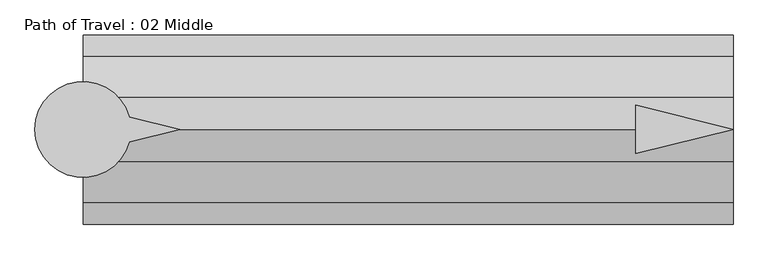
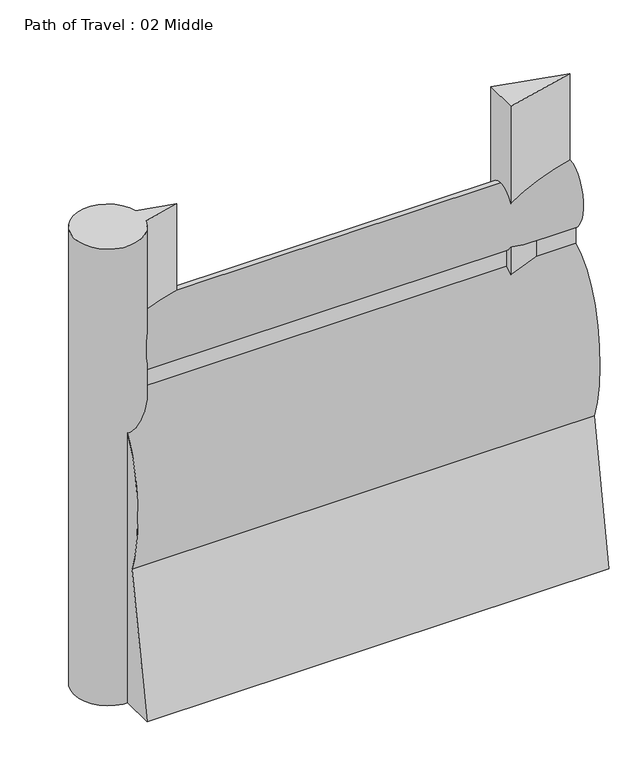
"""IFC4 building model written with IfcOpenShell, lengths in millimetres: proxy geometry, Path of Travel : 02 Middle."""

import ifcopenshell
import ifcopenshell.guid

model = None  # the IFC model being written
_history = None  # IfcOwnerHistory: only IFC2X3 demands one
_inside = {}  # id of a spatial element -> (the spatial element, [elements in it])
_under = {}  # id of a project, library or spatial element -> (it, [spatial elements below it])
_declared = {}  # id of a project -> (the project, [libraries it declares])
_typed = {}  # id of a type object -> (the type object, [elements of that type])
_made_of = {}  # id of a material, layer set ... -> (it, [elements and type objects made of it])


def new_model(schema):
    """Start an empty IFC model of exactly this schema.

    Asked for "IFC4X3", IfcOpenShell would pick the latest addendum, in which some entities
    have other attributes; the version numbers below select the first issue.
    IFC2X3 requires an IfcOwnerHistory on every rooted entity: one is made here for all.
    """
    global model, _history
    if schema == "IFC4X3":
        model = ifcopenshell.file(schema_version=(4, 3, 0, 0))
    else:
        model = ifcopenshell.file(schema=schema)
    _inside.clear()
    _under.clear()
    _declared.clear()
    _typed.clear()
    _made_of.clear()
    _history = None
    if model.schema == "IFC2X3":
        org = make("IfcOrganization", Name="unknown")
        user = make(
            "IfcPersonAndOrganization",
            ThePerson=make("IfcPerson", FamilyName="unknown"),
            TheOrganization=org,
        )
        app = make(
            "IfcApplication",
            ApplicationDeveloper=org,
            Version="unknown",
            ApplicationFullName="unknown",
            ApplicationIdentifier="unknown",
        )
        _history = make(
            "IfcOwnerHistory",
            OwningUser=user,
            OwningApplication=app,
            ChangeAction="ADDED",
            CreationDate=0,
        )
    return model


def make(cls, **values):
    """One entity of the class cls with the attributes given. An attribute that is None is left unset."""
    return model.create_entity(
        cls, **{name: value for name, value in values.items() if value is not None}
    )


def rooted(cls, **values):
    """An entity with a GlobalId (a new one), such as an element, a storey or a relation."""
    return make(cls, GlobalId=ifcopenshell.guid.new(), OwnerHistory=_history, **values)


def si_unit(unit_type, name, prefix=None):
    """IfcSIUnit, for example si_unit("LENGTHUNIT", "METRE", prefix="MILLI")."""
    return make("IfcSIUnit", UnitType=unit_type, Prefix=prefix, Name=name)


def assignment(units):
    """IfcUnitAssignment: the units of a project."""
    return None if units is None else make("IfcUnitAssignment", Units=units)


def point(xyz):
    """IfcCartesianPoint."""
    return None if xyz is None else make("IfcCartesianPoint", Coordinates=xyz)


def direction(xyz):
    """IfcDirection."""
    return None if xyz is None else make("IfcDirection", DirectionRatios=xyz)


def frame(location, z_axis=None, x_axis=None):
    """IfcAxis2Placement3D, a coordinate frame: its origin and axes. An axis left out is left unset."""
    return make(
        "IfcAxis2Placement3D",
        Location=point(location),
        Axis=direction(z_axis),
        RefDirection=direction(x_axis),
    )


def frame_2d(location, x_axis=None):
    """IfcAxis2Placement2D, a coordinate frame in the plane: its origin and x axis."""
    return make(
        "IfcAxis2Placement2D", Location=point(location), RefDirection=direction(x_axis)
    )


def origin():
    """The frame at (0, 0, 0) with its axes left unset."""
    return frame((0.0, 0.0, 0.0))


def origin_with_axes():
    """The frame at (0, 0, 0) with the z axis (0, 0, 1) and the x axis (1, 0, 0) written out."""
    return frame((0.0, 0.0, 0.0), z_axis=(0.0, 0.0, 1.0), x_axis=(1.0, 0.0, 0.0))


def place(relative_to, where):
    """IfcLocalPlacement: puts the frame where relative to a parent placement (None: the world)."""
    return make(
        "IfcLocalPlacement", PlacementRelTo=relative_to, RelativePlacement=where
    )


def context(
    kind, dimensions, precision=None, world=None, true_north=None, identifier=None
):
    """IfcGeometricRepresentationContext, for example the 3D "Model" context."""
    return make(
        "IfcGeometricRepresentationContext",
        ContextIdentifier=identifier,
        ContextType=kind,
        CoordinateSpaceDimension=dimensions,
        Precision=precision,
        WorldCoordinateSystem=world,
        TrueNorth=true_north,
    )


def project(units=None, contexts=None):
    """IfcProject with its units and contexts."""
    return rooted(
        "IfcProject",
        Name="project",
        RepresentationContexts=contexts,
        UnitsInContext=assignment(units),
    )


def spatial(cls, under=None, at=None, **own):
    """A site, building, storey or space (cls), placed at a placement, below another one or the project."""
    s = rooted(cls, ObjectPlacement=at, **own)
    if under is not None:
        _under.setdefault(under.id(), (under, []))[1].append(s)
    return s


def polyline(points):
    """IfcPolyline through the points."""
    return make("IfcPolyline", Points=[point(p) for p in points])


def circle_curve(where, radius):
    """IfcCircle in the frame where."""
    return make("IfcCircle", Position=where, Radius=radius)


def ellipse_curve(where, semi_axis1, semi_axis2):
    """IfcEllipse in the frame where."""
    return make(
        "IfcEllipse", Position=where, SemiAxis1=semi_axis1, SemiAxis2=semi_axis2
    )


def trimmed(basis, trim1, trim2, sense, master):
    """IfcTrimmedCurve: the piece of a basis curve between two trims."""
    return make(
        "IfcTrimmedCurve",
        BasisCurve=basis,
        Trim1=trim1,
        Trim2=trim2,
        SenseAgreement=sense,
        MasterRepresentation=master,
    )


def segment(curve, same_sense, transition):
    """IfcCompositeCurveSegment."""
    return make(
        "IfcCompositeCurveSegment",
        Transition=transition,
        SameSense=same_sense,
        ParentCurve=curve,
    )


def composite_curve(segments, self_intersect=None):
    """IfcCompositeCurve: segments joined end to end."""
    return make("IfcCompositeCurve", Segments=segments, SelfIntersect=self_intersect)


def outline(outer, holes=None, kind="AREA"):
    """IfcArbitraryClosedProfileDef: a profile drawn as a closed curve; with holes, ...WithVoids."""
    if holes is None:
        return make("IfcArbitraryClosedProfileDef", ProfileType=kind, OuterCurve=outer)
    return make(
        "IfcArbitraryProfileDefWithVoids",
        ProfileType=kind,
        OuterCurve=outer,
        InnerCurves=holes,
    )


def extrude(swept, where, along, depth):
    """IfcExtrudedAreaSolid: the profile swept, set in the frame where, extruded along a direction by depth."""
    return make(
        "IfcExtrudedAreaSolid",
        SweptArea=swept,
        Position=where,
        ExtrudedDirection=direction(along),
        Depth=depth,
    )


def shape(context_of_items, identifier, shape_type, items):
    """IfcShapeRepresentation: the items that make up one representation, for example the "Body"."""
    return make(
        "IfcShapeRepresentation",
        ContextOfItems=context_of_items,
        RepresentationIdentifier=identifier,
        RepresentationType=shape_type,
        Items=items,
    )


def source(mapping_origin, context_of_items, identifier, shape_type, items):
    """IfcRepresentationMap: a shape defined once, which mapped items show again and again."""
    return make(
        "IfcRepresentationMap",
        MappingOrigin=mapping_origin,
        MappedRepresentation=shape(context_of_items, identifier, shape_type, items),
    )


def transform(
    local_origin,
    x_axis=None,
    y_axis=None,
    z_axis=None,
    scale=None,
    scale2=None,
    scale3=None,
    uniform=True,
):
    """IfcCartesianTransformationOperator3D, or its non-uniform kind. x_axis, y_axis, z_axis: its Axis1, 2, 3."""
    if uniform:
        return make(
            "IfcCartesianTransformationOperator3D",
            Axis1=direction(x_axis),
            Axis2=direction(y_axis),
            LocalOrigin=point(local_origin),
            Scale=scale,
            Axis3=direction(z_axis),
        )
    return make(
        "IfcCartesianTransformationOperator3DnonUniform",
        Axis1=direction(x_axis),
        Axis2=direction(y_axis),
        LocalOrigin=point(local_origin),
        Scale=scale,
        Axis3=direction(z_axis),
        Scale2=scale2,
        Scale3=scale3,
    )


def mapped(mapping_source, mapping_target):
    """IfcMappedItem: shows the shape of a source again, moved by a transform."""
    return make(
        "IfcMappedItem", MappingSource=mapping_source, MappingTarget=mapping_target
    )


def made_of(thing, what):
    """Note that an element or type object is made of a material, layer set ...; save() writes the relation."""
    if what is not None:
        _made_of.setdefault(what.id(), (what, []))[1].append(thing)
    return thing


def element(
    cls,
    number,
    at=None,
    inside=None,
    cuts=None,
    type_object=None,
    material=None,
    context=None,
    identifier="Body",
    shape_type=None,
    held_by="IfcProductDefinitionShape",
    body=None,
    shapes=None,
    **own,
):
    """One element of the class cls, such as IfcWall. Its Tag is "e" and its number.

    at: its placement. inside: the storey or other place that contains it. cuts: it is an
    opening in that element (IfcRelVoidsElement). A single representation is given by context,
    identifier, shape_type and body (its items); several are given by shapes. held_by: the class
    of the entity that holds the representations. save() writes the other relations.
    """
    e = rooted(cls, Tag="e%d" % number, ObjectPlacement=at, **own)
    if body is not None:
        shapes = [shape(context, identifier, shape_type, body)]
    if shapes is not None:
        e.Representation = make(held_by, Representations=shapes)
    if inside is not None:
        _inside.setdefault(inside.id(), (inside, []))[1].append(e)
    if cuts is not None:
        rooted(
            "IfcRelVoidsElement", RelatingBuildingElement=cuts, RelatedOpeningElement=e
        )
    if type_object is not None:
        _typed.setdefault(type_object.id(), (type_object, []))[1].append(e)
    return made_of(e, material)


def aggregate(whole, parts):
    """IfcRelAggregates: a whole, such as a stair, and the parts it consists of."""
    return rooted("IfcRelAggregates", RelatingObject=whole, RelatedObjects=parts)


def save(model, path):
    """Write the relations noted so far, then the file.

    IfcRelAggregates (storeys below a building ...), IfcRelContainedInSpatialStructure (elements
    in a storey), IfcRelDefinesByType, IfcRelAssociatesMaterial and IfcRelDeclares: one each for
    every whole, place, type object, material and project.
    """
    for whole, parts in _under.values():
        aggregate(whole, parts)
    for where, things in _inside.values():
        rooted(
            "IfcRelContainedInSpatialStructure",
            RelatedElements=things,
            RelatingStructure=where,
        )
    for kind, things in _typed.values():
        rooted("IfcRelDefinesByType", RelatedObjects=things, RelatingType=kind)
    for what, things in _made_of.values():
        rooted("IfcRelAssociatesMaterial", RelatedObjects=things, RelatingMaterial=what)
    for by, libraries in _declared.values():
        rooted("IfcRelDeclares", RelatingContext=by, RelatedDefinitions=libraries)
    model.write(path)


def plane_surface(at):
    """IfcPlane: the flat surface through the origin of the frame at, square to its z axis."""
    return make("IfcPlane", Position=at)


def extruded_surface(curve, direction_of_extrusion, depth):
    """IfcSurfaceOfLinearExtrusion: the curve pushed along a direction by depth."""
    return make(
        "IfcSurfaceOfLinearExtrusion",
        SweptCurve=make("IfcArbitraryOpenProfileDef", ProfileType="CURVE", Curve=curve),
        ExtrudedDirection=direction(direction_of_extrusion),
        Depth=depth,
    )


def advanced_brep(points, edges, surfaces, faces):
    """IfcAdvancedBrep: a solid bounded by faces that lie on surfaces and meet in shared edges.

    An edge is (start, end): straight between two places in points (the first is 0);
    or (start, end, curve); or (start, end, curve, False) where it runs against its curve.
    A face is (place in surfaces, loops), or (place, loops, False) where it looks against
    its surface's normal. A loop lists edges by number (the first is 1), with a minus sign
    where the edge is run from its end to its start. The first loop is the outer one.
    """
    corners = [point(p) for p in points]
    vertices = [make("IfcVertexPoint", VertexGeometry=c) for c in corners]
    made = []
    for start, end, *more in edges:
        made.append(
            make(
                "IfcEdgeCurve",
                EdgeStart=vertices[start],
                EdgeEnd=vertices[end],
                EdgeGeometry=more[0] if more else make("IfcPolyline", Points=[corners[start], corners[end]]),
                SameSense=more[1] if len(more) > 1 else True,
            )
        )
    hull = []
    for where, loops, *sense in faces:
        bounds = []
        for j, loop in enumerate(loops):
            ring = [make("IfcOrientedEdge", EdgeElement=made[abs(k) - 1], Orientation=k > 0) for k in loop]
            bounds.append(
                make(
                    "IfcFaceOuterBound" if j == 0 else "IfcFaceBound",
                    Bound=make("IfcEdgeLoop", EdgeList=ring),
                    Orientation=True,
                )
            )
        hull.append(make("IfcAdvancedFace", Bounds=bounds, FaceSurface=surfaces[where], SameSense=sense[0] if sense else True))
    return make("IfcAdvancedBrep", Outer=make("IfcClosedShell", CfsFaces=hull))


def path_of_travel_02_middle_ae4c9040(model_context):
    return source(origin(), model_context, "Body", "SolidModel", [
        advanced_brep(
        [(227.5554837, 0.0, 1727.2), (227.5554837, 42.9018657, 1436.6534209), (227.5554837, 42.9018657, 1363.4763406), (227.5554837, 184.1186263, 643.4144547), (227.5554837, 297.5699544, 0.0), (227.5554837, 145.6574193, 0.0), (227.5554837, 0.0, 584.2), (227.5554837, -145.6574193, 0.0), (227.5554837, -297.5699544, 0.0), (227.5554837, -184.1186263, 643.4144547), (227.5554837, -42.9018657, 1363.4763406), (227.5554837, -42.9018657, 1436.6534209), (2268.4123179, 0.0, 1727.2), (2268.4123179, -42.9018657, 1436.6534209), (2268.4123179, -42.9018657, 1363.4763406), (2268.4123179, -184.1186263, 643.4144547), (2268.4123179, -297.5699544, 0.0), (2268.4123179, -145.6574193, 0.0), (2268.4123179, 0.0, 584.2), (2268.4123179, 145.6574193, 0.0), (2268.4123179, 297.5699544, 0.0), (2268.4123179, 184.1186263, 643.4144547), (2268.4123179, 42.9018657, 1363.4763406), (2268.4123179, 42.9018657, 1436.6534209)],
        [
            (0, 1, ellipse_curve(frame((227.5554837, 0.0, 1574.8), z_axis=(-1.0, 0.0, 0.0), x_axis=(0.0, 0.0, 1.0)), 152.4, 101.6)),
            (1, 2),
            (2, 3, ellipse_curve(frame((227.5554837, 0.0, 914.4), z_axis=(-1.0, 0.0, 0.0), x_axis=(0.0, 0.0, -1.0)), 457.2, 228.6)),
            (3, 4),
            (4, 5),
            (5, 6),
            (6, 7),
            (7, 8),
            (8, 9),
            (9, 10, ellipse_curve(frame((227.5554837, 0.0, 914.4), z_axis=(-1.0, 0.0, 0.0), x_axis=(0.0, 0.0, -1.0)), 457.2, 228.6)),
            (10, 11),
            (11, 0, ellipse_curve(frame((227.5554837, 0.0, 1574.8), z_axis=(-1.0, 0.0, 0.0), x_axis=(0.0, 0.0, 1.0)), 152.4, 101.6)),
            (12, 13, ellipse_curve(frame((2268.4123179, 0.0, 1574.8), z_axis=(1.0, 0.0, 0.0), x_axis=(0.0, 0.0, 1.0)), 152.4, 101.6)),
            (13, 14),
            (14, 15, ellipse_curve(frame((2268.4123179, 0.0, 914.4), z_axis=(1.0, 0.0, 0.0), x_axis=(0.0, 0.0, -1.0)), 457.2, 228.6)),
            (15, 16),
            (16, 17),
            (17, 18),
            (18, 19),
            (19, 20),
            (20, 21),
            (21, 22, ellipse_curve(frame((2268.4123179, 0.0, 914.4), z_axis=(1.0, 0.0, 0.0), x_axis=(0.0, 0.0, -1.0)), 457.2, 228.6)),
            (22, 23),
            (23, 12, ellipse_curve(frame((2268.4123179, 0.0, 1574.8), z_axis=(1.0, 0.0, 0.0), x_axis=(0.0, 0.0, 1.0)), 152.4, 101.6)),
            (0, 12),
            (23, 1),
            (22, 2),
            (21, 3),
            (20, 4),
            (19, 5),
            (18, 6),
            (17, 7),
            (16, 8),
            (15, 9),
            (14, 10),
            (13, 11),
        ],
        [
            plane_surface(frame((227.5554837, 0.0, 0.0), z_axis=(-1.0, 0.0, 0.0), x_axis=(0.0, 0.0, 1.0))),
            plane_surface(frame((2268.4123179, 0.0, 0.0), z_axis=(1.0, 0.0, 0.0), x_axis=(0.0, 0.0, 1.0))),
            extruded_surface(trimmed(ellipse_curve(frame((2268.4123179, 0.0, 1574.8), z_axis=(-1.0, 0.0, 0.0), x_axis=(0.0, 0.0, 1.0)), 152.4, 101.6), [point((2268.4123179, 0.0, 1727.2))], [point((2268.4123179, 42.9018657, 1436.6534209))], True, "CARTESIAN"), (-2040.8568341999999, 0.0, 0.0), 2040.8568341999999),
            plane_surface(frame((227.5554837, 42.9018657, 1436.6534209), z_axis=(0.0, 1.0, 0.0), x_axis=(1.0, 0.0, 0.0))),
            extruded_surface(trimmed(ellipse_curve(frame((2268.4123179, 0.0, 914.4), z_axis=(-1.0, 0.0, 0.0), x_axis=(0.0, 0.0, -1.0)), 457.2, 228.6), [point((2268.4123179, 42.9018657, 1363.4763406))], [point((2268.4123179, 184.1186263, 643.4144547))], True, "CARTESIAN"), (-2040.8568341999999, 0.0, 0.0), 2040.8568341999999),
            plane_surface(frame((227.5554837, 184.1186263, 643.4144547), z_axis=(0.0, 0.9848077530122078, 0.1736481776669322), x_axis=(1.0, 0.0, 0.0))),
            plane_surface(frame((227.5554837, 297.5699544, 0.0), z_axis=(0.0, 0.0, -1.0), x_axis=(1.0, 0.0, 0.0))),
            plane_surface(frame((227.5554837, 145.6574193, 0.0), z_axis=(0.0, -0.9702957262760199, -0.2419218955995739), x_axis=(1.0, 0.0, 0.0))),
            plane_surface(frame((227.5554837, 0.0, 584.2), z_axis=(0.0, 0.9702957262759961, -0.24192189559966923), x_axis=(1.0, 0.0, 0.0))),
            plane_surface(frame((227.5554837, -145.6574193, 0.0), z_axis=(0.0, 0.0, -1.0), x_axis=(1.0, 0.0, 0.0))),
            plane_surface(frame((227.5554837, -297.5699544, 0.0), z_axis=(0.0, -0.984807753012208, 0.17364817766693066), x_axis=(1.0, 0.0, 0.0))),
            extruded_surface(trimmed(ellipse_curve(frame((2268.4123179, 0.0, 914.4), z_axis=(-1.0, 0.0, 0.0), x_axis=(0.0, 0.0, -1.0)), 457.2, 228.6), [point((2268.4123179, -184.1186263, 643.4144547))], [point((2268.4123179, -42.9018657, 1363.4763406))], True, "CARTESIAN"), (-2040.8568341999999, 0.0, 0.0), 2040.8568341999999),
            plane_surface(frame((227.5554837, -42.9018657, 1363.4763406), z_axis=(0.0, -1.0, 0.0), x_axis=(1.0, 0.0, 0.0))),
            extruded_surface(trimmed(ellipse_curve(frame((2268.4123179, 0.0, 1574.8), z_axis=(-1.0, 0.0, 0.0), x_axis=(0.0, 0.0, 1.0)), 152.4, 101.6), [point((2268.4123179, -42.9018657, 1436.6534209))], [point((2268.4123179, 0.0, 1727.2))], True, "CARTESIAN"), (-2040.8568341999999, 0.0, 0.0), 2040.8568341999999),
        ],
        [
            (0, [[1, 2, 3, 4, 5, 6, 7, 8, 9, 10, 11, 12]]),
            (1, [[13, 14, 15, 16, 17, 18, 19, 20, 21, 22, 23, 24]]),
            (2, [[-1, 25, -24, 26]]),
            (3, [[-2, -26, -23, 27]]),
            (4, [[-3, -27, -22, 28]]),
            (5, [[-4, -28, -21, 29]]),
            (6, [[-5, -29, -20, 30]]),
            (7, [[-6, -30, -19, 31]]),
            (8, [[-7, -31, -18, 32]]),
            (9, [[-8, -32, -17, 33]]),
            (10, [[-9, -33, -16, 34]]),
            (11, [[-10, -34, -15, 35]]),
            (12, [[-11, -35, -14, 36]]),
            (13, [[-12, -36, -13, -25]]),
        ],
    ),
        extrude(outline(polyline([(1962.4071713, 76.2006338), (2268.4123179, 0.0), (1962.4071713, -76.2006338), (1962.4071713, 76.2006338)])), origin_with_axes(), (0.0, 0.0, 1.0), 2129.5973753),
        extrude(outline(composite_curve([segment(polyline([(372.7837828, 39.4440225), (531.182385, 0.0), (372.7837828, -39.4440225)]), True, "CONTINUOUS"), segment(trimmed(circle_curve(frame_2d((227.2200886, 0.0)), 150.8131956), [point((372.7837828, -39.4440225))], [point((372.7837828, 39.4440225))], False, "CARTESIAN"), True, "CONTINUOUS")], self_intersect=False)), origin_with_axes(), (0.0, 0.0, 1.0), 2129.5973753),
    ])


if __name__ == "__main__":
    model = new_model("IFC4")
    model_context = context("Model", 3, world=origin())
    ifc_project = project(units=[si_unit("LENGTHUNIT", "METRE", prefix="MILLI")], contexts=[model_context])
    site = spatial("IfcSite", under=ifc_project)
    building = spatial("IfcBuilding", under=site)
    placement = place(None, origin())
    path_of_travel_02_middle_shape = path_of_travel_02_middle_ae4c9040(model_context)
    element("IfcBuildingElementProxy", 1, Name="Path of Travel : 02 Middle", ObjectType="Path of Travel : 02 Middle", at=placement, inside=building, context=model_context, shape_type="MappedRepresentation", body=[
        mapped(path_of_travel_02_middle_shape, transform((0.0, 0.0, 0.0), x_axis=(1.0, 0.0, 0.0), y_axis=(0.0, 1.0, 0.0), z_axis=(0.0, 0.0, 1.0))),
    ])
    save(model, "model.ifc")

# Revit data of these elements
# Type "Path of Travel : 02 Middle"
#   Path of Egress [instance default] = 4' - 0"
#   built-in parameter 1001306 [instance default] = 4 (stored number, unit not read)
#   Dot at Start = no
#   Arrow in Middle = yes
#   Arrow at End = no
#   Egress Path = none
# Element 1 (IfcBuildingElementProxy, "Path of Travel : 02 Middle")
#   Path of Egress = 6' - 8.34869"
#   built-in parameter 1001306 = 6.69572 (stored number, unit not read)
#   Materials on its faces: "Egress Path Solid", "solid"
# Materials
#   "Egress Path Solid": class "Unassigned", colour RGB 255 128 64, transparency 0.75, Comments = "Rendering appearance not upgraded "
#   "solid": class "Generic", colour RGB 120 120 120, transparency 0, Cost = 0
